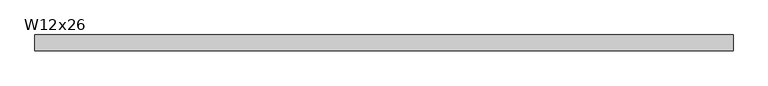
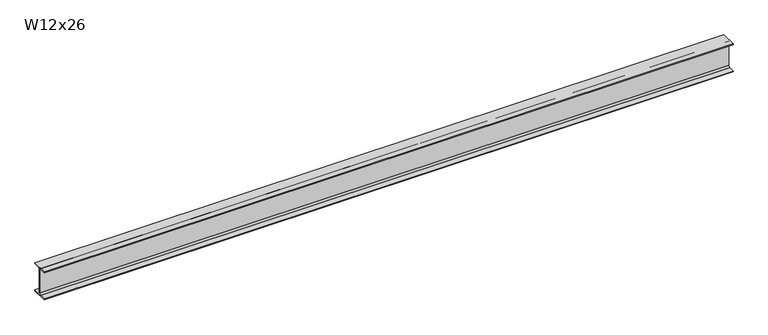
"""IFC4 building model written with IfcOpenShell, lengths in millimetres: beam geometry, RME W-Wide Flange : W12x26."""

from ifc_helpers import new_model, si_unit, point, frame, frame_2d, origin, place, context, project, spatial, polyline, circle_curve, trimmed, segment, composite_curve, outline, extrude, source, transform, mapped, element, save


def w12x26_d5a462bc(model_context):
    return source(origin(), model_context, "Body", "SweptSolid", [
        extrude(outline(composite_curve([segment(polyline([(82.423, -145.288), (82.423, -154.94), (-82.423, -154.94), (-82.423, -145.288), (-20.2565, -145.288)]), True, "CONTINUOUS"), segment(trimmed(circle_curve(frame_2d((-20.2565, -127.9525)), 17.3355), [point((-20.2565, -145.288))], [point((-2.921, -127.9525))], True, "CARTESIAN"), True, "CONTINUOUS"), segment(polyline([(-2.921, -127.9525), (-2.921, 127.9525)]), True, "CONTINUOUS"), segment(trimmed(circle_curve(frame_2d((-20.2565, 127.9525)), 17.3355), [point((-2.921, 127.9525))], [point((-20.2565, 145.288))], True, "CARTESIAN"), True, "CONTINUOUS"), segment(polyline([(-20.2565, 145.288), (-82.423, 145.288), (-82.423, 154.94), (82.423, 154.94), (82.423, 145.288), (20.2565, 145.288)]), True, "CONTINUOUS"), segment(trimmed(circle_curve(frame_2d((20.2565, 127.9525)), 17.3355), [point((20.2565, 145.288))], [point((2.921, 127.9525))], True, "CARTESIAN"), True, "CONTINUOUS"), segment(polyline([(2.921, 127.9525), (2.921, -127.9525)]), True, "CONTINUOUS"), segment(trimmed(circle_curve(frame_2d((20.2565, -127.9525)), 17.3355), [point((2.921, -127.9525))], [point((20.2565, -145.288))], True, "CARTESIAN"), True, "CONTINUOUS"), segment(polyline([(20.2565, -145.288), (82.423, -145.288)]), True, "CONTINUOUS")], self_intersect=False)), frame((-3587.75, 0.0, 0.0), z_axis=(1.0, 0.0, 0.0), x_axis=(0.0, 1.0, 0.0)), (0.0, 0.0, 1.0), 7207.123),
    ])


if __name__ == "__main__":
    model = new_model("IFC4")
    model_context = context("Model", 3, world=origin())
    ifc_project = project(units=[si_unit("LENGTHUNIT", "METRE", prefix="MILLI")], contexts=[model_context])
    site = spatial("IfcSite", under=ifc_project)
    building = spatial("IfcBuilding", under=site)
    placement = place(None, origin())
    w12x26_shape = w12x26_d5a462bc(model_context)
    element("IfcBeam", 1, ObjectType="RME W-Wide Flange : W12x26", at=placement, inside=building, context=model_context, shape_type="MappedRepresentation", body=[
        mapped(w12x26_shape, transform((0.0, 0.0, 0.0), x_axis=(1.0, 0.0, 0.0), y_axis=(0.0, 1.0, 0.0), z_axis=(0.0, 0.0, 1.0))),
    ])
    save(model, "model.ifc")

# Revit data of these elements
# Type "RME W-Wide Flange : W12x26"
#   WELD P [instance default] = ""
#   WELD LE [instance default] = ""
#   WELD D [instance default] = ""
#   TOP SECTION SIZE [instance default] = ""
#   TOP SECTION LENGTH [instance default] = ""
#   REMARKS [instance default] = ""
#   REINF TYPE [instance default] = ""
#   Nominal Size = "W24"
#   End Bearing Capacity [instance default] = ""
#   BOT SECTION SIZE [instance default] = ""
#   BOT SECTION LENGTH [instance default] = ""
#   Assembly Code = "B10"
#   W = 26
#   Start Extension Calculation [instance default] = 10' - 0"
#   Start Extension [instance default] = -0' - 0 1/2"
#   End Extension Calculation [instance default] = 10' - 0"
#   End Extension [instance default] = -0' - 0 1/2"
#   Length [instance default] = 5' - 0"
#   bf = 0' - 6.49"
#   d = 1' - 0.2"
#   k = 0' - 1 1/16"
#   k2 = 0' - 0.6825"
#   tf = 0' - 0.38"
#   tw = 0' - 0.23"
#   A = 0.053125 SF
#   Structural Material [instance default] = Metal - Steel - ASTM A992
# Element 1 (IfcBeam, "RME W-Wide Flange : W12x26")
#   Length = 24' - 2"
#   Materials on its faces: "Metal - Steel - ASTM A992"
# Materials
#   "Metal - Steel - ASTM A992": class "Metal", colour RGB 255 128 0, transparency 0
